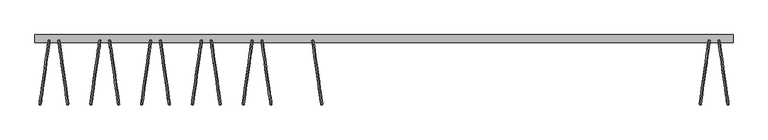
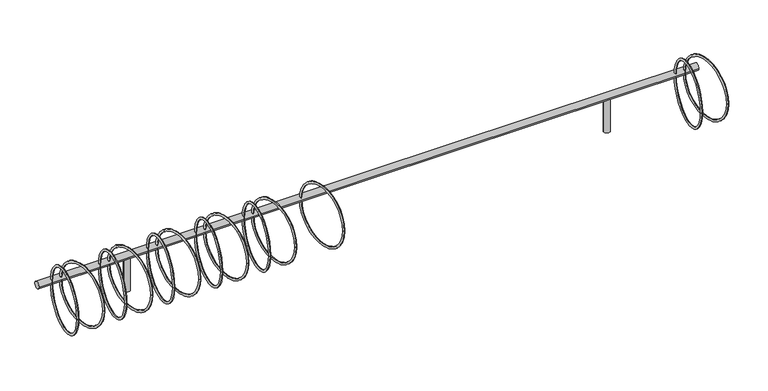
"""IFC4 building model written with IfcOpenShell, lengths in millimetres: geographic element geometry, NLRS_90_SI_WPB_fietsenrek staal_gen_bf : fietsenrek 5500mm 14 plaatsen."""

from ifc_helpers import new_model, si_unit, point, frame, frame_2d, origin, origin_with_axes, place, context, project, spatial, circle_curve, ellipse_curve, trimmed, segment, composite_curve, outline, extrude, source, transform, mapped, element, save
from ifc_brep_helpers import revolved_surface, advanced_brep


def geographic_element_d13230c3(model_context):
    return source(origin(), model_context, "Body", "SolidModel", [
        advanced_brep(
        [(-560.5888305, -21.9255981, 304.7993564), (-492.0982681, -509.2612714, 304.7993564), (-489.8888952, -524.981777, 304.7993564), (-562.7982034, -6.2050925, 304.7993564)],
        [
            (0, 1, circle_curve(frame((-526.3435493, -265.5934347, 304.7993564), z_axis=(0.9902680687415715, 0.1391731009600577, 0.0), x_axis=(0.1391731009600577, -0.9902680687415715, 0.0)), 246.0625)),
            (1, 2, circle_curve(frame((-490.9935817, -517.1215242, 304.7993564), z_axis=(0.0, 0.0, 1.0), x_axis=(-0.13917310096005775, 0.9902680687415715, 0.0)), 7.9375)),
            (2, 3, circle_curve(frame((-526.3435493, -265.5934347, 304.7993564), z_axis=(-0.9902680687415715, -0.1391731009600577, 0.0), x_axis=(0.1391731009600577, -0.9902680687415715, 0.0)), 261.9375)),
            (3, 0, circle_curve(frame((-561.6935169, -14.0653453, 304.7993564), z_axis=(0.0, 0.0, 1.0), x_axis=(0.13917310096005764, -0.9902680687415715, 0.0)), 7.9375)),
            (2, 1, circle_curve(frame((-490.9935817, -517.1215242, 304.7993564), z_axis=(0.0, 0.0, 1.0), x_axis=(-0.13917310096005775, 0.9902680687415715, 0.0)), 7.9375)),
            (0, 3, circle_curve(frame((-561.6935169, -14.0653453, 304.7993564), z_axis=(0.0, 0.0, 1.0), x_axis=(0.13917310096005764, -0.9902680687415715, 0.0)), 7.9375)),
            (1, 0, circle_curve(frame((-526.3435493, -265.5934347, 304.7993564), z_axis=(0.9902680687415715, 0.1391731009600577, 0.0), x_axis=(-0.1391731009600577, 0.9902680687415715, 0.0)), 246.0625)),
            (3, 2, circle_curve(frame((-526.3435493, -265.5934347, 304.7993564), z_axis=(-0.9902680687415715, -0.1391731009600577, 0.0), x_axis=(-0.1391731009600577, 0.9902680687415715, 0.0)), 261.9375)),
        ],
        [
            revolved_surface(trimmed(ellipse_curve(frame((-490.9935817, -517.1215242, 304.7993564), z_axis=(0.0, 0.0, -1.0), x_axis=(-0.13917310096005775, 0.9902680687415715, 0.0)), 7.9375, 7.9375), [point((-489.8888952, -524.981777, 304.7993564))], [point((-492.0982681, -509.2612714, 304.7993564))], True, "CARTESIAN"), (-714.9896164, -292.1059105, 304.7993564), (-0.9902680687415715, -0.1391731009600577, 0.0)),
            revolved_surface(trimmed(ellipse_curve(frame((-490.9935817, -517.1215242, 304.7993564), z_axis=(0.0, 0.0, -1.0), x_axis=(-0.13917310096005775, 0.9902680687415715, 0.0)), 7.9375, 7.9375), [point((-492.0982681, -509.2612714, 304.7993564))], [point((-489.8888952, -524.981777, 304.7993564))], True, "CARTESIAN"), (-714.9896164, -292.1059105, 304.7993564), (-0.9902680687415715, -0.1391731009600577, 0.0)),
            revolved_surface(trimmed(ellipse_curve(frame((-561.6935169, -14.0653453, 304.7993564), z_axis=(0.0, 0.0, 1.0), x_axis=(0.1391731009600577, -0.9902680687415715, 0.0)), 7.9375, 7.9375), [point((-562.7982034, -6.2050925, 304.7993564))], [point((-560.5888305, -21.9255981, 304.7993564))], True, "CARTESIAN"), (-714.9896164, -292.1059105, 304.7993564), (-0.9902680687415715, -0.1391731009600577, 0.0)),
            revolved_surface(trimmed(ellipse_curve(frame((-561.6935169, -14.0653453, 304.7993564), z_axis=(0.0, 0.0, 1.0), x_axis=(0.1391731009600577, -0.9902680687415715, 0.0)), 7.9375, 7.9375), [point((-560.5888305, -21.9255981, 304.7993564))], [point((-562.7982034, -6.2050925, 304.7993564))], True, "CARTESIAN"), (-714.9896164, -292.1059105, 304.7993564), (-0.9902680687415715, -0.1391731009600577, 0.0)),
        ],
        [
            (0, [[1, 2, 3, 4]]),
            (1, [[-3, 5, -1, 6]]),
            (2, [[7, -4, 8, -2]]),
            (3, [[-8, -6, -7, -5]]),
        ],
    ),
        advanced_brep(
        [(-1039.4111695, -21.9255981, 304.7993564), (-1107.9017319, -509.2612714, 304.7993564), (-1110.1111048, -524.981777, 304.7993564), (-1037.2017966, -6.2050925, 304.7993564)],
        [
            (0, 1, circle_curve(frame((-1073.6564507, -265.5934347, 304.7993564), z_axis=(0.990268068741571, -0.13917310096006058, 0.0), x_axis=(-0.13917310096006058, -0.990268068741571, 0.0)), 246.0625)),
            (1, 2, circle_curve(frame((-1109.0064183, -517.1215242, 304.7993564), z_axis=(0.0, 0.0, 1.0), x_axis=(0.13917310096006055, 0.990268068741571, 0.0)), 7.9375)),
            (2, 3, circle_curve(frame((-1073.6564507, -265.5934347, 304.7993564), z_axis=(-0.990268068741571, 0.13917310096006058, 0.0), x_axis=(-0.13917310096006058, -0.990268068741571, 0.0)), 261.9375)),
            (3, 0, circle_curve(frame((-1038.3064831, -14.0653453, 304.7993564), z_axis=(0.0, 0.0, 1.0), x_axis=(-0.1391731009600606, -0.990268068741571, 0.0)), 7.9375)),
            (2, 1, circle_curve(frame((-1109.0064183, -517.1215242, 304.7993564), z_axis=(0.0, 0.0, 1.0), x_axis=(0.13917310096006055, 0.990268068741571, 0.0)), 7.9375)),
            (0, 3, circle_curve(frame((-1038.3064831, -14.0653453, 304.7993564), z_axis=(0.0, 0.0, 1.0), x_axis=(-0.1391731009600606, -0.990268068741571, 0.0)), 7.9375)),
            (1, 0, circle_curve(frame((-1073.6564507, -265.5934347, 304.7993564), z_axis=(0.990268068741571, -0.13917310096006058, 0.0), x_axis=(0.13917310096006058, 0.990268068741571, 0.0)), 246.0625)),
            (3, 2, circle_curve(frame((-1073.6564507, -265.5934347, 304.7993564), z_axis=(-0.990268068741571, 0.13917310096006058, 0.0), x_axis=(0.13917310096006058, 0.990268068741571, 0.0)), 261.9375)),
        ],
        [
            revolved_surface(trimmed(ellipse_curve(frame((-1109.0064183, -517.1215242, 304.7993564), z_axis=(0.0, 0.0, -1.0), x_axis=(0.13917310096006055, 0.990268068741571, 0.0)), 7.9375, 7.9375), [point((-1110.1111048, -524.981777, 304.7993564))], [point((-1107.9017319, -509.2612714, 304.7993564))], True, "CARTESIAN"), (-885.0103836, -292.1059105, 304.7993564), (-0.990268068741571, 0.13917310096006058, 0.0)),
            revolved_surface(trimmed(ellipse_curve(frame((-1109.0064183, -517.1215242, 304.7993564), z_axis=(0.0, 0.0, -1.0), x_axis=(0.13917310096006055, 0.990268068741571, 0.0)), 7.9375, 7.9375), [point((-1107.9017319, -509.2612714, 304.7993564))], [point((-1110.1111048, -524.981777, 304.7993564))], True, "CARTESIAN"), (-885.0103836, -292.1059105, 304.7993564), (-0.990268068741571, 0.13917310096006058, 0.0)),
            revolved_surface(trimmed(ellipse_curve(frame((-1038.3064831, -14.0653453, 304.7993564), z_axis=(0.0, 0.0, 1.0), x_axis=(-0.13917310096006055, -0.990268068741571, 0.0)), 7.9375, 7.9375), [point((-1037.2017966, -6.2050925, 304.7993564))], [point((-1039.4111695, -21.9255981, 304.7993564))], True, "CARTESIAN"), (-885.0103836, -292.1059105, 304.7993564), (-0.990268068741571, 0.13917310096006058, 0.0)),
            revolved_surface(trimmed(ellipse_curve(frame((-1038.3064831, -14.0653453, 304.7993564), z_axis=(0.0, 0.0, 1.0), x_axis=(-0.13917310096006055, -0.990268068741571, 0.0)), 7.9375, 7.9375), [point((-1039.4111695, -21.9255981, 304.7993564))], [point((-1037.2017966, -6.2050925, 304.7993564))], True, "CARTESIAN"), (-885.0103836, -292.1059105, 304.7993564), (-0.990268068741571, 0.13917310096006058, 0.0)),
        ],
        [
            (0, [[1, 2, 3, 4]]),
            (1, [[-3, 5, -1, 6]]),
            (2, [[7, -4, 8, -2]]),
            (3, [[-8, -6, -7, -5]]),
        ],
    ),
        advanced_brep(
        [(-960.5888305, -21.9255981, 304.7993564), (-892.0982681, -509.2612714, 304.7993564), (-889.8888952, -524.981777, 304.7993564), (-962.7982034, -6.2050925, 304.7993564)],
        [
            (0, 1, circle_curve(frame((-926.3435493, -265.5934347, 304.7993564), z_axis=(0.9902680687415715, 0.1391731009600577, 0.0), x_axis=(0.1391731009600577, -0.9902680687415715, 0.0)), 246.0625)),
            (1, 2, circle_curve(frame((-890.9935817, -517.1215242, 304.7993564), z_axis=(0.0, 0.0, 1.0), x_axis=(-0.13917310096005775, 0.9902680687415715, 0.0)), 7.9375)),
            (2, 3, circle_curve(frame((-926.3435493, -265.5934347, 304.7993564), z_axis=(-0.9902680687415715, -0.1391731009600577, 0.0), x_axis=(0.1391731009600577, -0.9902680687415715, 0.0)), 261.9375)),
            (3, 0, circle_curve(frame((-961.6935169, -14.0653453, 304.7993564), z_axis=(0.0, 0.0, 1.0), x_axis=(0.13917310096005764, -0.9902680687415715, 0.0)), 7.9375)),
            (2, 1, circle_curve(frame((-890.9935817, -517.1215242, 304.7993564), z_axis=(0.0, 0.0, 1.0), x_axis=(-0.13917310096005775, 0.9902680687415715, 0.0)), 7.9375)),
            (0, 3, circle_curve(frame((-961.6935169, -14.0653453, 304.7993564), z_axis=(0.0, 0.0, 1.0), x_axis=(0.13917310096005764, -0.9902680687415715, 0.0)), 7.9375)),
            (1, 0, circle_curve(frame((-926.3435493, -265.5934347, 304.7993564), z_axis=(0.9902680687415715, 0.1391731009600577, 0.0), x_axis=(-0.1391731009600577, 0.9902680687415715, 0.0)), 246.0625)),
            (3, 2, circle_curve(frame((-926.3435493, -265.5934347, 304.7993564), z_axis=(-0.9902680687415715, -0.1391731009600577, 0.0), x_axis=(-0.1391731009600577, 0.9902680687415715, 0.0)), 261.9375)),
        ],
        [
            revolved_surface(trimmed(ellipse_curve(frame((-890.9935817, -517.1215242, 304.7993564), z_axis=(0.0, 0.0, -1.0), x_axis=(-0.13917310096005775, 0.9902680687415715, 0.0)), 7.9375, 7.9375), [point((-889.8888952, -524.981777, 304.7993564))], [point((-892.0982681, -509.2612714, 304.7993564))], True, "CARTESIAN"), (-1114.9896164, -292.1059105, 304.7993564), (-0.9902680687415715, -0.1391731009600577, 0.0)),
            revolved_surface(trimmed(ellipse_curve(frame((-890.9935817, -517.1215242, 304.7993564), z_axis=(0.0, 0.0, -1.0), x_axis=(-0.13917310096005775, 0.9902680687415715, 0.0)), 7.9375, 7.9375), [point((-892.0982681, -509.2612714, 304.7993564))], [point((-889.8888952, -524.981777, 304.7993564))], True, "CARTESIAN"), (-1114.9896164, -292.1059105, 304.7993564), (-0.9902680687415715, -0.1391731009600577, 0.0)),
            revolved_surface(trimmed(ellipse_curve(frame((-961.6935169, -14.0653453, 304.7993564), z_axis=(0.0, 0.0, 1.0), x_axis=(0.1391731009600577, -0.9902680687415715, 0.0)), 7.9375, 7.9375), [point((-962.7982034, -6.2050925, 304.7993564))], [point((-960.5888305, -21.9255981, 304.7993564))], True, "CARTESIAN"), (-1114.9896164, -292.1059105, 304.7993564), (-0.9902680687415715, -0.1391731009600577, 0.0)),
            revolved_surface(trimmed(ellipse_curve(frame((-961.6935169, -14.0653453, 304.7993564), z_axis=(0.0, 0.0, 1.0), x_axis=(0.1391731009600577, -0.9902680687415715, 0.0)), 7.9375, 7.9375), [point((-960.5888305, -21.9255981, 304.7993564))], [point((-962.7982034, -6.2050925, 304.7993564))], True, "CARTESIAN"), (-1114.9896164, -292.1059105, 304.7993564), (-0.9902680687415715, -0.1391731009600577, 0.0)),
        ],
        [
            (0, [[1, 2, 3, 4]]),
            (1, [[-3, 5, -1, 6]]),
            (2, [[7, -4, 8, -2]]),
            (3, [[-8, -6, -7, -5]]),
        ],
    ),
        advanced_brep(
        [(-1439.4111695, -21.9255981, 304.7993564), (-1507.9017319, -509.2612714, 304.7993564), (-1510.1111048, -524.981777, 304.7993564), (-1437.2017966, -6.2050925, 304.7993564)],
        [
            (0, 1, circle_curve(frame((-1473.6564507, -265.5934347, 304.7993564), z_axis=(0.990268068741571, -0.13917310096006058, 0.0), x_axis=(-0.13917310096006058, -0.990268068741571, 0.0)), 246.0625)),
            (1, 2, circle_curve(frame((-1509.0064183, -517.1215242, 304.7993564), z_axis=(0.0, 0.0, 1.0), x_axis=(0.13917310096006055, 0.990268068741571, 0.0)), 7.9375)),
            (2, 3, circle_curve(frame((-1473.6564507, -265.5934347, 304.7993564), z_axis=(-0.990268068741571, 0.13917310096006058, 0.0), x_axis=(-0.13917310096006058, -0.990268068741571, 0.0)), 261.9375)),
            (3, 0, circle_curve(frame((-1438.3064831, -14.0653453, 304.7993564), z_axis=(0.0, 0.0, 1.0), x_axis=(-0.1391731009600606, -0.990268068741571, 0.0)), 7.9375)),
            (2, 1, circle_curve(frame((-1509.0064183, -517.1215242, 304.7993564), z_axis=(0.0, 0.0, 1.0), x_axis=(0.13917310096006055, 0.990268068741571, 0.0)), 7.9375)),
            (0, 3, circle_curve(frame((-1438.3064831, -14.0653453, 304.7993564), z_axis=(0.0, 0.0, 1.0), x_axis=(-0.1391731009600606, -0.990268068741571, 0.0)), 7.9375)),
            (1, 0, circle_curve(frame((-1473.6564507, -265.5934347, 304.7993564), z_axis=(0.990268068741571, -0.13917310096006058, 0.0), x_axis=(0.13917310096006058, 0.990268068741571, 0.0)), 246.0625)),
            (3, 2, circle_curve(frame((-1473.6564507, -265.5934347, 304.7993564), z_axis=(-0.990268068741571, 0.13917310096006058, 0.0), x_axis=(0.13917310096006058, 0.990268068741571, 0.0)), 261.9375)),
        ],
        [
            revolved_surface(trimmed(ellipse_curve(frame((-1509.0064183, -517.1215242, 304.7993564), z_axis=(0.0, 0.0, -1.0), x_axis=(0.13917310096006055, 0.990268068741571, 0.0)), 7.9375, 7.9375), [point((-1510.1111048, -524.981777, 304.7993564))], [point((-1507.9017319, -509.2612714, 304.7993564))], True, "CARTESIAN"), (-1285.0103836, -292.1059105, 304.7993564), (-0.990268068741571, 0.13917310096006058, 0.0)),
            revolved_surface(trimmed(ellipse_curve(frame((-1509.0064183, -517.1215242, 304.7993564), z_axis=(0.0, 0.0, -1.0), x_axis=(0.13917310096006055, 0.990268068741571, 0.0)), 7.9375, 7.9375), [point((-1507.9017319, -509.2612714, 304.7993564))], [point((-1510.1111048, -524.981777, 304.7993564))], True, "CARTESIAN"), (-1285.0103836, -292.1059105, 304.7993564), (-0.990268068741571, 0.13917310096006058, 0.0)),
            revolved_surface(trimmed(ellipse_curve(frame((-1438.3064831, -14.0653453, 304.7993564), z_axis=(0.0, 0.0, 1.0), x_axis=(-0.13917310096006055, -0.990268068741571, 0.0)), 7.9375, 7.9375), [point((-1437.2017966, -6.2050925, 304.7993564))], [point((-1439.4111695, -21.9255981, 304.7993564))], True, "CARTESIAN"), (-1285.0103836, -292.1059105, 304.7993564), (-0.990268068741571, 0.13917310096006058, 0.0)),
            revolved_surface(trimmed(ellipse_curve(frame((-1438.3064831, -14.0653453, 304.7993564), z_axis=(0.0, 0.0, 1.0), x_axis=(-0.13917310096006055, -0.990268068741571, 0.0)), 7.9375, 7.9375), [point((-1439.4111695, -21.9255981, 304.7993564))], [point((-1437.2017966, -6.2050925, 304.7993564))], True, "CARTESIAN"), (-1285.0103836, -292.1059105, 304.7993564), (-0.990268068741571, 0.13917310096006058, 0.0)),
        ],
        [
            (0, [[1, 2, 3, 4]]),
            (1, [[-3, 5, -1, 6]]),
            (2, [[7, -4, 8, -2]]),
            (3, [[-8, -6, -7, -5]]),
        ],
    ),
        advanced_brep(
        [(-1360.5888305, -21.9255981, 304.7993564), (-1292.0982681, -509.2612714, 304.7993564), (-1289.8888952, -524.981777, 304.7993564), (-1362.7982034, -6.2050925, 304.7993564)],
        [
            (0, 1, circle_curve(frame((-1326.3435493, -265.5934347, 304.7993564), z_axis=(0.9902680687415715, 0.1391731009600577, 0.0), x_axis=(0.1391731009600577, -0.9902680687415715, 0.0)), 246.0625)),
            (1, 2, circle_curve(frame((-1290.9935817, -517.1215242, 304.7993564), z_axis=(0.0, 0.0, 1.0), x_axis=(-0.13917310096005775, 0.9902680687415715, 0.0)), 7.9375)),
            (2, 3, circle_curve(frame((-1326.3435493, -265.5934347, 304.7993564), z_axis=(-0.9902680687415715, -0.1391731009600577, 0.0), x_axis=(0.1391731009600577, -0.9902680687415715, 0.0)), 261.9375)),
            (3, 0, circle_curve(frame((-1361.6935169, -14.0653453, 304.7993564), z_axis=(0.0, 0.0, 1.0), x_axis=(0.13917310096005764, -0.9902680687415715, 0.0)), 7.9375)),
            (2, 1, circle_curve(frame((-1290.9935817, -517.1215242, 304.7993564), z_axis=(0.0, 0.0, 1.0), x_axis=(-0.13917310096005775, 0.9902680687415715, 0.0)), 7.9375)),
            (0, 3, circle_curve(frame((-1361.6935169, -14.0653453, 304.7993564), z_axis=(0.0, 0.0, 1.0), x_axis=(0.13917310096005764, -0.9902680687415715, 0.0)), 7.9375)),
            (1, 0, circle_curve(frame((-1326.3435493, -265.5934347, 304.7993564), z_axis=(0.9902680687415715, 0.1391731009600577, 0.0), x_axis=(-0.1391731009600577, 0.9902680687415715, 0.0)), 246.0625)),
            (3, 2, circle_curve(frame((-1326.3435493, -265.5934347, 304.7993564), z_axis=(-0.9902680687415715, -0.1391731009600577, 0.0), x_axis=(-0.1391731009600577, 0.9902680687415715, 0.0)), 261.9375)),
        ],
        [
            revolved_surface(trimmed(ellipse_curve(frame((-1290.9935817, -517.1215242, 304.7993564), z_axis=(0.0, 0.0, -1.0), x_axis=(-0.13917310096005775, 0.9902680687415715, 0.0)), 7.9375, 7.9375), [point((-1289.8888952, -524.981777, 304.7993564))], [point((-1292.0982681, -509.2612714, 304.7993564))], True, "CARTESIAN"), (-1514.9896164, -292.1059105, 304.7993564), (-0.9902680687415715, -0.1391731009600577, 0.0)),
            revolved_surface(trimmed(ellipse_curve(frame((-1290.9935817, -517.1215242, 304.7993564), z_axis=(0.0, 0.0, -1.0), x_axis=(-0.13917310096005775, 0.9902680687415715, 0.0)), 7.9375, 7.9375), [point((-1292.0982681, -509.2612714, 304.7993564))], [point((-1289.8888952, -524.981777, 304.7993564))], True, "CARTESIAN"), (-1514.9896164, -292.1059105, 304.7993564), (-0.9902680687415715, -0.1391731009600577, 0.0)),
            revolved_surface(trimmed(ellipse_curve(frame((-1361.6935169, -14.0653453, 304.7993564), z_axis=(0.0, 0.0, 1.0), x_axis=(0.1391731009600577, -0.9902680687415715, 0.0)), 7.9375, 7.9375), [point((-1362.7982034, -6.2050925, 304.7993564))], [point((-1360.5888305, -21.9255981, 304.7993564))], True, "CARTESIAN"), (-1514.9896164, -292.1059105, 304.7993564), (-0.9902680687415715, -0.1391731009600577, 0.0)),
            revolved_surface(trimmed(ellipse_curve(frame((-1361.6935169, -14.0653453, 304.7993564), z_axis=(0.0, 0.0, 1.0), x_axis=(0.1391731009600577, -0.9902680687415715, 0.0)), 7.9375, 7.9375), [point((-1360.5888305, -21.9255981, 304.7993564))], [point((-1362.7982034, -6.2050925, 304.7993564))], True, "CARTESIAN"), (-1514.9896164, -292.1059105, 304.7993564), (-0.9902680687415715, -0.1391731009600577, 0.0)),
        ],
        [
            (0, [[1, 2, 3, 4]]),
            (1, [[-3, 5, -1, 6]]),
            (2, [[7, -4, 8, -2]]),
            (3, [[-8, -6, -7, -5]]),
        ],
    ),
        advanced_brep(
        [(-1839.4111695, -21.9255981, 304.7993564), (-1907.9017319, -509.2612714, 304.7993564), (-1910.1111048, -524.981777, 304.7993564), (-1837.2017966, -6.2050925, 304.7993564)],
        [
            (0, 1, circle_curve(frame((-1873.6564507, -265.5934347, 304.7993564), z_axis=(0.990268068741571, -0.13917310096006058, 0.0), x_axis=(-0.13917310096006058, -0.990268068741571, 0.0)), 246.0625)),
            (1, 2, circle_curve(frame((-1909.0064183, -517.1215242, 304.7993564), z_axis=(0.0, 0.0, 1.0), x_axis=(0.13917310096006055, 0.990268068741571, 0.0)), 7.9375)),
            (2, 3, circle_curve(frame((-1873.6564507, -265.5934347, 304.7993564), z_axis=(-0.990268068741571, 0.13917310096006058, 0.0), x_axis=(-0.13917310096006058, -0.990268068741571, 0.0)), 261.9375)),
            (3, 0, circle_curve(frame((-1838.3064831, -14.0653453, 304.7993564), z_axis=(0.0, 0.0, 1.0), x_axis=(-0.1391731009600606, -0.990268068741571, 0.0)), 7.9375)),
            (2, 1, circle_curve(frame((-1909.0064183, -517.1215242, 304.7993564), z_axis=(0.0, 0.0, 1.0), x_axis=(0.13917310096006055, 0.990268068741571, 0.0)), 7.9375)),
            (0, 3, circle_curve(frame((-1838.3064831, -14.0653453, 304.7993564), z_axis=(0.0, 0.0, 1.0), x_axis=(-0.1391731009600606, -0.990268068741571, 0.0)), 7.9375)),
            (1, 0, circle_curve(frame((-1873.6564507, -265.5934347, 304.7993564), z_axis=(0.990268068741571, -0.13917310096006058, 0.0), x_axis=(0.13917310096006058, 0.990268068741571, 0.0)), 246.0625)),
            (3, 2, circle_curve(frame((-1873.6564507, -265.5934347, 304.7993564), z_axis=(-0.990268068741571, 0.13917310096006058, 0.0), x_axis=(0.13917310096006058, 0.990268068741571, 0.0)), 261.9375)),
        ],
        [
            revolved_surface(trimmed(ellipse_curve(frame((-1909.0064183, -517.1215242, 304.7993564), z_axis=(0.0, 0.0, -1.0), x_axis=(0.13917310096006055, 0.990268068741571, 0.0)), 7.9375, 7.9375), [point((-1910.1111048, -524.981777, 304.7993564))], [point((-1907.9017319, -509.2612714, 304.7993564))], True, "CARTESIAN"), (-1685.0103836, -292.1059105, 304.7993564), (-0.990268068741571, 0.13917310096006058, 0.0)),
            revolved_surface(trimmed(ellipse_curve(frame((-1909.0064183, -517.1215242, 304.7993564), z_axis=(0.0, 0.0, -1.0), x_axis=(0.13917310096006055, 0.990268068741571, 0.0)), 7.9375, 7.9375), [point((-1907.9017319, -509.2612714, 304.7993564))], [point((-1910.1111048, -524.981777, 304.7993564))], True, "CARTESIAN"), (-1685.0103836, -292.1059105, 304.7993564), (-0.990268068741571, 0.13917310096006058, 0.0)),
            revolved_surface(trimmed(ellipse_curve(frame((-1838.3064831, -14.0653453, 304.7993564), z_axis=(0.0, 0.0, 1.0), x_axis=(-0.13917310096006055, -0.990268068741571, 0.0)), 7.9375, 7.9375), [point((-1837.2017966, -6.2050925, 304.7993564))], [point((-1839.4111695, -21.9255981, 304.7993564))], True, "CARTESIAN"), (-1685.0103836, -292.1059105, 304.7993564), (-0.990268068741571, 0.13917310096006058, 0.0)),
            revolved_surface(trimmed(ellipse_curve(frame((-1838.3064831, -14.0653453, 304.7993564), z_axis=(0.0, 0.0, 1.0), x_axis=(-0.13917310096006055, -0.990268068741571, 0.0)), 7.9375, 7.9375), [point((-1839.4111695, -21.9255981, 304.7993564))], [point((-1837.2017966, -6.2050925, 304.7993564))], True, "CARTESIAN"), (-1685.0103836, -292.1059105, 304.7993564), (-0.990268068741571, 0.13917310096006058, 0.0)),
        ],
        [
            (0, [[1, 2, 3, 4]]),
            (1, [[-3, 5, -1, 6]]),
            (2, [[7, -4, 8, -2]]),
            (3, [[-8, -6, -7, -5]]),
        ],
    ),
        advanced_brep(
        [(-1760.5888305, -21.9255981, 304.7993564), (-1692.0982681, -509.2612714, 304.7993564), (-1689.8888952, -524.981777, 304.7993564), (-1762.7982034, -6.2050925, 304.7993564)],
        [
            (0, 1, circle_curve(frame((-1726.3435493, -265.5934347, 304.7993564), z_axis=(0.9902680687415715, 0.1391731009600577, 0.0), x_axis=(0.1391731009600577, -0.9902680687415715, 0.0)), 246.0625)),
            (1, 2, circle_curve(frame((-1690.9935817, -517.1215242, 304.7993564), z_axis=(0.0, 0.0, 1.0), x_axis=(-0.13917310096005775, 0.9902680687415715, 0.0)), 7.9375)),
            (2, 3, circle_curve(frame((-1726.3435493, -265.5934347, 304.7993564), z_axis=(-0.9902680687415715, -0.1391731009600577, 0.0), x_axis=(0.1391731009600577, -0.9902680687415715, 0.0)), 261.9375)),
            (3, 0, circle_curve(frame((-1761.6935169, -14.0653453, 304.7993564), z_axis=(0.0, 0.0, 1.0), x_axis=(0.13917310096005764, -0.9902680687415715, 0.0)), 7.9375)),
            (2, 1, circle_curve(frame((-1690.9935817, -517.1215242, 304.7993564), z_axis=(0.0, 0.0, 1.0), x_axis=(-0.13917310096005775, 0.9902680687415715, 0.0)), 7.9375)),
            (0, 3, circle_curve(frame((-1761.6935169, -14.0653453, 304.7993564), z_axis=(0.0, 0.0, 1.0), x_axis=(0.13917310096005764, -0.9902680687415715, 0.0)), 7.9375)),
            (1, 0, circle_curve(frame((-1726.3435493, -265.5934347, 304.7993564), z_axis=(0.9902680687415715, 0.1391731009600577, 0.0), x_axis=(-0.1391731009600577, 0.9902680687415715, 0.0)), 246.0625)),
            (3, 2, circle_curve(frame((-1726.3435493, -265.5934347, 304.7993564), z_axis=(-0.9902680687415715, -0.1391731009600577, 0.0), x_axis=(-0.1391731009600577, 0.9902680687415715, 0.0)), 261.9375)),
        ],
        [
            revolved_surface(trimmed(ellipse_curve(frame((-1690.9935817, -517.1215242, 304.7993564), z_axis=(0.0, 0.0, -1.0), x_axis=(-0.13917310096005775, 0.9902680687415715, 0.0)), 7.9375, 7.9375), [point((-1689.8888952, -524.981777, 304.7993564))], [point((-1692.0982681, -509.2612714, 304.7993564))], True, "CARTESIAN"), (-1914.9896164, -292.1059105, 304.7993564), (-0.9902680687415715, -0.1391731009600577, 0.0)),
            revolved_surface(trimmed(ellipse_curve(frame((-1690.9935817, -517.1215242, 304.7993564), z_axis=(0.0, 0.0, -1.0), x_axis=(-0.13917310096005775, 0.9902680687415715, 0.0)), 7.9375, 7.9375), [point((-1692.0982681, -509.2612714, 304.7993564))], [point((-1689.8888952, -524.981777, 304.7993564))], True, "CARTESIAN"), (-1914.9896164, -292.1059105, 304.7993564), (-0.9902680687415715, -0.1391731009600577, 0.0)),
            revolved_surface(trimmed(ellipse_curve(frame((-1761.6935169, -14.0653453, 304.7993564), z_axis=(0.0, 0.0, 1.0), x_axis=(0.1391731009600577, -0.9902680687415715, 0.0)), 7.9375, 7.9375), [point((-1762.7982034, -6.2050925, 304.7993564))], [point((-1760.5888305, -21.9255981, 304.7993564))], True, "CARTESIAN"), (-1914.9896164, -292.1059105, 304.7993564), (-0.9902680687415715, -0.1391731009600577, 0.0)),
            revolved_surface(trimmed(ellipse_curve(frame((-1761.6935169, -14.0653453, 304.7993564), z_axis=(0.0, 0.0, 1.0), x_axis=(0.1391731009600577, -0.9902680687415715, 0.0)), 7.9375, 7.9375), [point((-1760.5888305, -21.9255981, 304.7993564))], [point((-1762.7982034, -6.2050925, 304.7993564))], True, "CARTESIAN"), (-1914.9896164, -292.1059105, 304.7993564), (-0.9902680687415715, -0.1391731009600577, 0.0)),
        ],
        [
            (0, [[1, 2, 3, 4]]),
            (1, [[-3, 5, -1, 6]]),
            (2, [[7, -4, 8, -2]]),
            (3, [[-8, -6, -7, -5]]),
        ],
    ),
        advanced_brep(
        [(-2239.4111695, -21.9255981, 304.7993564), (-2307.9017319, -509.2612714, 304.7993564), (-2310.1111048, -524.981777, 304.7993564), (-2237.2017966, -6.2050925, 304.7993564)],
        [
            (0, 1, circle_curve(frame((-2273.6564507, -265.5934347, 304.7993564), z_axis=(0.990268068741571, -0.13917310096006058, 0.0), x_axis=(-0.13917310096006058, -0.990268068741571, 0.0)), 246.0625)),
            (1, 2, circle_curve(frame((-2309.0064183, -517.1215242, 304.7993564), z_axis=(0.0, 0.0, 1.0), x_axis=(0.13917310096006055, 0.990268068741571, 0.0)), 7.9375)),
            (2, 3, circle_curve(frame((-2273.6564507, -265.5934347, 304.7993564), z_axis=(-0.990268068741571, 0.13917310096006058, 0.0), x_axis=(-0.13917310096006058, -0.990268068741571, 0.0)), 261.9375)),
            (3, 0, circle_curve(frame((-2238.3064831, -14.0653453, 304.7993564), z_axis=(0.0, 0.0, 1.0), x_axis=(-0.1391731009600606, -0.990268068741571, 0.0)), 7.9375)),
            (2, 1, circle_curve(frame((-2309.0064183, -517.1215242, 304.7993564), z_axis=(0.0, 0.0, 1.0), x_axis=(0.13917310096006055, 0.990268068741571, 0.0)), 7.9375)),
            (0, 3, circle_curve(frame((-2238.3064831, -14.0653453, 304.7993564), z_axis=(0.0, 0.0, 1.0), x_axis=(-0.1391731009600606, -0.990268068741571, 0.0)), 7.9375)),
            (1, 0, circle_curve(frame((-2273.6564507, -265.5934347, 304.7993564), z_axis=(0.990268068741571, -0.13917310096006058, 0.0), x_axis=(0.13917310096006058, 0.990268068741571, 0.0)), 246.0625)),
            (3, 2, circle_curve(frame((-2273.6564507, -265.5934347, 304.7993564), z_axis=(-0.990268068741571, 0.13917310096006058, 0.0), x_axis=(0.13917310096006058, 0.990268068741571, 0.0)), 261.9375)),
        ],
        [
            revolved_surface(trimmed(ellipse_curve(frame((-2309.0064183, -517.1215242, 304.7993564), z_axis=(0.0, 0.0, -1.0), x_axis=(0.13917310096006055, 0.990268068741571, 0.0)), 7.9375, 7.9375), [point((-2310.1111048, -524.981777, 304.7993564))], [point((-2307.9017319, -509.2612714, 304.7993564))], True, "CARTESIAN"), (-2085.0103836, -292.1059105, 304.7993564), (-0.990268068741571, 0.13917310096006058, 0.0)),
            revolved_surface(trimmed(ellipse_curve(frame((-2309.0064183, -517.1215242, 304.7993564), z_axis=(0.0, 0.0, -1.0), x_axis=(0.13917310096006055, 0.990268068741571, 0.0)), 7.9375, 7.9375), [point((-2307.9017319, -509.2612714, 304.7993564))], [point((-2310.1111048, -524.981777, 304.7993564))], True, "CARTESIAN"), (-2085.0103836, -292.1059105, 304.7993564), (-0.990268068741571, 0.13917310096006058, 0.0)),
            revolved_surface(trimmed(ellipse_curve(frame((-2238.3064831, -14.0653453, 304.7993564), z_axis=(0.0, 0.0, 1.0), x_axis=(-0.13917310096006055, -0.990268068741571, 0.0)), 7.9375, 7.9375), [point((-2237.2017966, -6.2050925, 304.7993564))], [point((-2239.4111695, -21.9255981, 304.7993564))], True, "CARTESIAN"), (-2085.0103836, -292.1059105, 304.7993564), (-0.990268068741571, 0.13917310096006058, 0.0)),
            revolved_surface(trimmed(ellipse_curve(frame((-2238.3064831, -14.0653453, 304.7993564), z_axis=(0.0, 0.0, 1.0), x_axis=(-0.13917310096006055, -0.990268068741571, 0.0)), 7.9375, 7.9375), [point((-2239.4111695, -21.9255981, 304.7993564))], [point((-2237.2017966, -6.2050925, 304.7993564))], True, "CARTESIAN"), (-2085.0103836, -292.1059105, 304.7993564), (-0.990268068741571, 0.13917310096006058, 0.0)),
        ],
        [
            (0, [[1, 2, 3, 4]]),
            (1, [[-3, 5, -1, 6]]),
            (2, [[7, -4, 8, -2]]),
            (3, [[-8, -6, -7, -5]]),
        ],
    ),
        advanced_brep(
        [(-2160.5888305, -21.9255981, 304.7993564), (-2092.0982681, -509.2612714, 304.7993564), (-2089.8888952, -524.981777, 304.7993564), (-2162.7982034, -6.2050925, 304.7993564)],
        [
            (0, 1, circle_curve(frame((-2126.3435493, -265.5934347, 304.7993564), z_axis=(0.9902680687415715, 0.1391731009600577, 0.0), x_axis=(0.1391731009600577, -0.9902680687415715, 0.0)), 246.0625)),
            (1, 2, circle_curve(frame((-2090.9935817, -517.1215242, 304.7993564), z_axis=(0.0, 0.0, 1.0), x_axis=(-0.13917310096005775, 0.9902680687415715, 0.0)), 7.9375)),
            (2, 3, circle_curve(frame((-2126.3435493, -265.5934347, 304.7993564), z_axis=(-0.9902680687415715, -0.1391731009600577, 0.0), x_axis=(0.1391731009600577, -0.9902680687415715, 0.0)), 261.9375)),
            (3, 0, circle_curve(frame((-2161.6935169, -14.0653453, 304.7993564), z_axis=(0.0, 0.0, 1.0), x_axis=(0.13917310096005764, -0.9902680687415715, 0.0)), 7.9375)),
            (2, 1, circle_curve(frame((-2090.9935817, -517.1215242, 304.7993564), z_axis=(0.0, 0.0, 1.0), x_axis=(-0.13917310096005775, 0.9902680687415715, 0.0)), 7.9375)),
            (0, 3, circle_curve(frame((-2161.6935169, -14.0653453, 304.7993564), z_axis=(0.0, 0.0, 1.0), x_axis=(0.13917310096005764, -0.9902680687415715, 0.0)), 7.9375)),
            (1, 0, circle_curve(frame((-2126.3435493, -265.5934347, 304.7993564), z_axis=(0.9902680687415715, 0.1391731009600577, 0.0), x_axis=(-0.1391731009600577, 0.9902680687415715, 0.0)), 246.0625)),
            (3, 2, circle_curve(frame((-2126.3435493, -265.5934347, 304.7993564), z_axis=(-0.9902680687415715, -0.1391731009600577, 0.0), x_axis=(-0.1391731009600577, 0.9902680687415715, 0.0)), 261.9375)),
        ],
        [
            revolved_surface(trimmed(ellipse_curve(frame((-2090.9935817, -517.1215242, 304.7993564), z_axis=(0.0, 0.0, -1.0), x_axis=(-0.13917310096005775, 0.9902680687415715, 0.0)), 7.9375, 7.9375), [point((-2089.8888952, -524.981777, 304.7993564))], [point((-2092.0982681, -509.2612714, 304.7993564))], True, "CARTESIAN"), (-2314.9896164, -292.1059105, 304.7993564), (-0.9902680687415715, -0.1391731009600577, 0.0)),
            revolved_surface(trimmed(ellipse_curve(frame((-2090.9935817, -517.1215242, 304.7993564), z_axis=(0.0, 0.0, -1.0), x_axis=(-0.13917310096005775, 0.9902680687415715, 0.0)), 7.9375, 7.9375), [point((-2092.0982681, -509.2612714, 304.7993564))], [point((-2089.8888952, -524.981777, 304.7993564))], True, "CARTESIAN"), (-2314.9896164, -292.1059105, 304.7993564), (-0.9902680687415715, -0.1391731009600577, 0.0)),
            revolved_surface(trimmed(ellipse_curve(frame((-2161.6935169, -14.0653453, 304.7993564), z_axis=(0.0, 0.0, 1.0), x_axis=(0.1391731009600577, -0.9902680687415715, 0.0)), 7.9375, 7.9375), [point((-2162.7982034, -6.2050925, 304.7993564))], [point((-2160.5888305, -21.9255981, 304.7993564))], True, "CARTESIAN"), (-2314.9896164, -292.1059105, 304.7993564), (-0.9902680687415715, -0.1391731009600577, 0.0)),
            revolved_surface(trimmed(ellipse_curve(frame((-2161.6935169, -14.0653453, 304.7993564), z_axis=(0.0, 0.0, 1.0), x_axis=(0.1391731009600577, -0.9902680687415715, 0.0)), 7.9375, 7.9375), [point((-2160.5888305, -21.9255981, 304.7993564))], [point((-2162.7982034, -6.2050925, 304.7993564))], True, "CARTESIAN"), (-2314.9896164, -292.1059105, 304.7993564), (-0.9902680687415715, -0.1391731009600577, 0.0)),
        ],
        [
            (0, [[1, 2, 3, 4]]),
            (1, [[-3, 5, -1, 6]]),
            (2, [[7, -4, 8, -2]]),
            (3, [[-8, -6, -7, -5]]),
        ],
    ),
        advanced_brep(
        [(2560.5888305, -21.9255981, 304.7993564), (2492.0982681, -509.2612714, 304.7993564), (2489.8888952, -524.981777, 304.7993564), (2562.7982034, -6.2050925, 304.7993564)],
        [
            (0, 1, circle_curve(frame((2526.3435493, -265.5934347, 304.7993564), z_axis=(0.990268068741571, -0.13917310096006058, 0.0), x_axis=(-0.13917310096006058, -0.990268068741571, 0.0)), 246.0625)),
            (1, 2, circle_curve(frame((2490.9935817, -517.1215242, 304.7993564), z_axis=(0.0, 0.0, 1.0), x_axis=(0.13917310096006055, 0.990268068741571, 0.0)), 7.9375)),
            (2, 3, circle_curve(frame((2526.3435493, -265.5934347, 304.7993564), z_axis=(-0.990268068741571, 0.13917310096006058, 0.0), x_axis=(-0.13917310096006058, -0.990268068741571, 0.0)), 261.9375)),
            (3, 0, circle_curve(frame((2561.6935169, -14.0653453, 304.7993564), z_axis=(0.0, 0.0, 1.0), x_axis=(-0.1391731009600606, -0.990268068741571, 0.0)), 7.9375)),
            (2, 1, circle_curve(frame((2490.9935817, -517.1215242, 304.7993564), z_axis=(0.0, 0.0, 1.0), x_axis=(0.13917310096006055, 0.990268068741571, 0.0)), 7.9375)),
            (0, 3, circle_curve(frame((2561.6935169, -14.0653453, 304.7993564), z_axis=(0.0, 0.0, 1.0), x_axis=(-0.1391731009600606, -0.990268068741571, 0.0)), 7.9375)),
            (1, 0, circle_curve(frame((2526.3435493, -265.5934347, 304.7993564), z_axis=(0.990268068741571, -0.13917310096006058, 0.0), x_axis=(0.13917310096006058, 0.990268068741571, 0.0)), 246.0625)),
            (3, 2, circle_curve(frame((2526.3435493, -265.5934347, 304.7993564), z_axis=(-0.990268068741571, 0.13917310096006058, 0.0), x_axis=(0.13917310096006058, 0.990268068741571, 0.0)), 261.9375)),
        ],
        [
            revolved_surface(trimmed(ellipse_curve(frame((2490.9935817, -517.1215242, 304.7993564), z_axis=(0.0, 0.0, -1.0), x_axis=(0.13917310096006055, 0.990268068741571, 0.0)), 7.9375, 7.9375), [point((2489.8888952, -524.981777, 304.7993564))], [point((2492.0982681, -509.2612714, 304.7993564))], True, "CARTESIAN"), (2714.9896164, -292.1059105, 304.7993564), (-0.990268068741571, 0.13917310096006058, 0.0)),
            revolved_surface(trimmed(ellipse_curve(frame((2490.9935817, -517.1215242, 304.7993564), z_axis=(0.0, 0.0, -1.0), x_axis=(0.13917310096006055, 0.990268068741571, 0.0)), 7.9375, 7.9375), [point((2492.0982681, -509.2612714, 304.7993564))], [point((2489.8888952, -524.981777, 304.7993564))], True, "CARTESIAN"), (2714.9896164, -292.1059105, 304.7993564), (-0.990268068741571, 0.13917310096006058, 0.0)),
            revolved_surface(trimmed(ellipse_curve(frame((2561.6935169, -14.0653453, 304.7993564), z_axis=(0.0, 0.0, 1.0), x_axis=(-0.13917310096006055, -0.990268068741571, 0.0)), 7.9375, 7.9375), [point((2562.7982034, -6.2050925, 304.7993564))], [point((2560.5888305, -21.9255981, 304.7993564))], True, "CARTESIAN"), (2714.9896164, -292.1059105, 304.7993564), (-0.990268068741571, 0.13917310096006058, 0.0)),
            revolved_surface(trimmed(ellipse_curve(frame((2561.6935169, -14.0653453, 304.7993564), z_axis=(0.0, 0.0, 1.0), x_axis=(-0.13917310096006055, -0.990268068741571, 0.0)), 7.9375, 7.9375), [point((2560.5888305, -21.9255981, 304.7993564))], [point((2562.7982034, -6.2050925, 304.7993564))], True, "CARTESIAN"), (2714.9896164, -292.1059105, 304.7993564), (-0.990268068741571, 0.13917310096006058, 0.0)),
        ],
        [
            (0, [[1, 2, 3, 4]]),
            (1, [[-3, 5, -1, 6]]),
            (2, [[7, -4, 8, -2]]),
            (3, [[-8, -6, -7, -5]]),
        ],
    ),
        advanced_brep(
        [(2639.4111695, -21.9255981, 304.7993564), (2707.9017319, -509.2612714, 304.7993564), (2710.1111048, -524.981777, 304.7993564), (2637.2017966, -6.2050925, 304.7993564)],
        [
            (0, 1, circle_curve(frame((2673.6564507, -265.5934347, 304.7993564), z_axis=(0.9902680687415715, 0.1391731009600577, 0.0), x_axis=(0.1391731009600577, -0.9902680687415715, 0.0)), 246.0625)),
            (1, 2, circle_curve(frame((2709.0064183, -517.1215242, 304.7993564), z_axis=(0.0, 0.0, 1.0), x_axis=(-0.13917310096005775, 0.9902680687415715, 0.0)), 7.9375)),
            (2, 3, circle_curve(frame((2673.6564507, -265.5934347, 304.7993564), z_axis=(-0.9902680687415715, -0.1391731009600577, 0.0), x_axis=(0.1391731009600577, -0.9902680687415715, 0.0)), 261.9375)),
            (3, 0, circle_curve(frame((2638.3064831, -14.0653453, 304.7993564), z_axis=(0.0, 0.0, 1.0), x_axis=(0.13917310096005764, -0.9902680687415715, 0.0)), 7.9375)),
            (2, 1, circle_curve(frame((2709.0064183, -517.1215242, 304.7993564), z_axis=(0.0, 0.0, 1.0), x_axis=(-0.13917310096005775, 0.9902680687415715, 0.0)), 7.9375)),
            (0, 3, circle_curve(frame((2638.3064831, -14.0653453, 304.7993564), z_axis=(0.0, 0.0, 1.0), x_axis=(0.13917310096005764, -0.9902680687415715, 0.0)), 7.9375)),
            (1, 0, circle_curve(frame((2673.6564507, -265.5934347, 304.7993564), z_axis=(0.9902680687415715, 0.1391731009600577, 0.0), x_axis=(-0.1391731009600577, 0.9902680687415715, 0.0)), 246.0625)),
            (3, 2, circle_curve(frame((2673.6564507, -265.5934347, 304.7993564), z_axis=(-0.9902680687415715, -0.1391731009600577, 0.0), x_axis=(-0.1391731009600577, 0.9902680687415715, 0.0)), 261.9375)),
        ],
        [
            revolved_surface(trimmed(ellipse_curve(frame((2709.0064183, -517.1215242, 304.7993564), z_axis=(0.0, 0.0, -1.0), x_axis=(-0.13917310096005775, 0.9902680687415715, 0.0)), 7.9375, 7.9375), [point((2710.1111048, -524.981777, 304.7993564))], [point((2707.9017319, -509.2612714, 304.7993564))], True, "CARTESIAN"), (2485.0103836, -292.1059105, 304.7993564), (-0.9902680687415715, -0.1391731009600577, 0.0)),
            revolved_surface(trimmed(ellipse_curve(frame((2709.0064183, -517.1215242, 304.7993564), z_axis=(0.0, 0.0, -1.0), x_axis=(-0.13917310096005775, 0.9902680687415715, 0.0)), 7.9375, 7.9375), [point((2707.9017319, -509.2612714, 304.7993564))], [point((2710.1111048, -524.981777, 304.7993564))], True, "CARTESIAN"), (2485.0103836, -292.1059105, 304.7993564), (-0.9902680687415715, -0.1391731009600577, 0.0)),
            revolved_surface(trimmed(ellipse_curve(frame((2638.3064831, -14.0653453, 304.7993564), z_axis=(0.0, 0.0, 1.0), x_axis=(0.1391731009600577, -0.9902680687415715, 0.0)), 7.9375, 7.9375), [point((2637.2017966, -6.2050925, 304.7993564))], [point((2639.4111695, -21.9255981, 304.7993564))], True, "CARTESIAN"), (2485.0103836, -292.1059105, 304.7993564), (-0.9902680687415715, -0.1391731009600577, 0.0)),
            revolved_surface(trimmed(ellipse_curve(frame((2638.3064831, -14.0653453, 304.7993564), z_axis=(0.0, 0.0, 1.0), x_axis=(0.1391731009600577, -0.9902680687415715, 0.0)), 7.9375, 7.9375), [point((2639.4111695, -21.9255981, 304.7993564))], [point((2637.2017966, -6.2050925, 304.7993564))], True, "CARTESIAN"), (2485.0103836, -292.1059105, 304.7993564), (-0.9902680687415715, -0.1391731009600577, 0.0)),
        ],
        [
            (0, [[1, 2, 3, 4]]),
            (1, [[-3, 5, -1, 6]]),
            (2, [[7, -4, 8, -2]]),
            (3, [[-8, -6, -7, -5]]),
        ],
    ),
        advanced_brep(
        [(-2639.4111695, -21.9255981, 304.7993564), (-2707.9017319, -509.2612714, 304.7993564), (-2710.1111048, -524.981777, 304.7993564), (-2637.2017966, -6.2050925, 304.7993564)],
        [
            (0, 1, circle_curve(frame((-2673.6564507, -265.5934347, 304.7993564), z_axis=(0.990268068741571, -0.13917310096006058, 0.0), x_axis=(-0.13917310096006058, -0.990268068741571, 0.0)), 246.0625)),
            (1, 2, circle_curve(frame((-2709.0064183, -517.1215242, 304.7993564), z_axis=(0.0, 0.0, 1.0), x_axis=(0.13917310096006055, 0.990268068741571, 0.0)), 7.9375)),
            (2, 3, circle_curve(frame((-2673.6564507, -265.5934347, 304.7993564), z_axis=(-0.990268068741571, 0.13917310096006058, 0.0), x_axis=(-0.13917310096006058, -0.990268068741571, 0.0)), 261.9375)),
            (3, 0, circle_curve(frame((-2638.3064831, -14.0653453, 304.7993564), z_axis=(0.0, 0.0, 1.0), x_axis=(-0.1391731009600606, -0.990268068741571, 0.0)), 7.9375)),
            (2, 1, circle_curve(frame((-2709.0064183, -517.1215242, 304.7993564), z_axis=(0.0, 0.0, 1.0), x_axis=(0.13917310096006055, 0.990268068741571, 0.0)), 7.9375)),
            (0, 3, circle_curve(frame((-2638.3064831, -14.0653453, 304.7993564), z_axis=(0.0, 0.0, 1.0), x_axis=(-0.1391731009600606, -0.990268068741571, 0.0)), 7.9375)),
            (1, 0, circle_curve(frame((-2673.6564507, -265.5934347, 304.7993564), z_axis=(0.990268068741571, -0.13917310096006058, 0.0), x_axis=(0.13917310096006058, 0.990268068741571, 0.0)), 246.0625)),
            (3, 2, circle_curve(frame((-2673.6564507, -265.5934347, 304.7993564), z_axis=(-0.990268068741571, 0.13917310096006058, 0.0), x_axis=(0.13917310096006058, 0.990268068741571, 0.0)), 261.9375)),
        ],
        [
            revolved_surface(trimmed(ellipse_curve(frame((-2709.0064183, -517.1215242, 304.7993564), z_axis=(0.0, 0.0, -1.0), x_axis=(0.13917310096006055, 0.990268068741571, 0.0)), 7.9375, 7.9375), [point((-2710.1111048, -524.981777, 304.7993564))], [point((-2707.9017319, -509.2612714, 304.7993564))], True, "CARTESIAN"), (-2485.0103836, -292.1059105, 304.7993564), (-0.990268068741571, 0.13917310096006058, 0.0)),
            revolved_surface(trimmed(ellipse_curve(frame((-2709.0064183, -517.1215242, 304.7993564), z_axis=(0.0, 0.0, -1.0), x_axis=(0.13917310096006055, 0.990268068741571, 0.0)), 7.9375, 7.9375), [point((-2707.9017319, -509.2612714, 304.7993564))], [point((-2710.1111048, -524.981777, 304.7993564))], True, "CARTESIAN"), (-2485.0103836, -292.1059105, 304.7993564), (-0.990268068741571, 0.13917310096006058, 0.0)),
            revolved_surface(trimmed(ellipse_curve(frame((-2638.3064831, -14.0653453, 304.7993564), z_axis=(0.0, 0.0, 1.0), x_axis=(-0.13917310096006055, -0.990268068741571, 0.0)), 7.9375, 7.9375), [point((-2637.2017966, -6.2050925, 304.7993564))], [point((-2639.4111695, -21.9255981, 304.7993564))], True, "CARTESIAN"), (-2485.0103836, -292.1059105, 304.7993564), (-0.990268068741571, 0.13917310096006058, 0.0)),
            revolved_surface(trimmed(ellipse_curve(frame((-2638.3064831, -14.0653453, 304.7993564), z_axis=(0.0, 0.0, 1.0), x_axis=(-0.13917310096006055, -0.990268068741571, 0.0)), 7.9375, 7.9375), [point((-2639.4111695, -21.9255981, 304.7993564))], [point((-2637.2017966, -6.2050925, 304.7993564))], True, "CARTESIAN"), (-2485.0103836, -292.1059105, 304.7993564), (-0.990268068741571, 0.13917310096006058, 0.0)),
        ],
        [
            (0, [[1, 2, 3, 4]]),
            (1, [[-3, 5, -1, 6]]),
            (2, [[7, -4, 8, -2]]),
            (3, [[-8, -6, -7, -5]]),
        ],
    ),
        advanced_brep(
        [(-2560.5888305, -21.9255981, 304.7993564), (-2492.0982681, -509.2612714, 304.7993564), (-2489.8888952, -524.981777, 304.7993564), (-2562.7982034, -6.2050925, 304.7993564)],
        [
            (0, 1, circle_curve(frame((-2526.3435493, -265.5934347, 304.7993564), z_axis=(0.9902680687415715, 0.1391731009600577, 0.0), x_axis=(0.1391731009600577, -0.9902680687415715, 0.0)), 246.0625)),
            (1, 2, circle_curve(frame((-2490.9935817, -517.1215242, 304.7993564), z_axis=(0.0, 0.0, 1.0), x_axis=(-0.13917310096005775, 0.9902680687415715, 0.0)), 7.9375)),
            (2, 3, circle_curve(frame((-2526.3435493, -265.5934347, 304.7993564), z_axis=(-0.9902680687415715, -0.1391731009600577, 0.0), x_axis=(0.1391731009600577, -0.9902680687415715, 0.0)), 261.9375)),
            (3, 0, circle_curve(frame((-2561.6935169, -14.0653453, 304.7993564), z_axis=(0.0, 0.0, 1.0), x_axis=(0.13917310096005764, -0.9902680687415715, 0.0)), 7.9375)),
            (2, 1, circle_curve(frame((-2490.9935817, -517.1215242, 304.7993564), z_axis=(0.0, 0.0, 1.0), x_axis=(-0.13917310096005775, 0.9902680687415715, 0.0)), 7.9375)),
            (0, 3, circle_curve(frame((-2561.6935169, -14.0653453, 304.7993564), z_axis=(0.0, 0.0, 1.0), x_axis=(0.13917310096005764, -0.9902680687415715, 0.0)), 7.9375)),
            (1, 0, circle_curve(frame((-2526.3435493, -265.5934347, 304.7993564), z_axis=(0.9902680687415715, 0.1391731009600577, 0.0), x_axis=(-0.1391731009600577, 0.9902680687415715, 0.0)), 246.0625)),
            (3, 2, circle_curve(frame((-2526.3435493, -265.5934347, 304.7993564), z_axis=(-0.9902680687415715, -0.1391731009600577, 0.0), x_axis=(-0.1391731009600577, 0.9902680687415715, 0.0)), 261.9375)),
        ],
        [
            revolved_surface(trimmed(ellipse_curve(frame((-2490.9935817, -517.1215242, 304.7993564), z_axis=(0.0, 0.0, -1.0), x_axis=(-0.13917310096005775, 0.9902680687415715, 0.0)), 7.9375, 7.9375), [point((-2489.8888952, -524.981777, 304.7993564))], [point((-2492.0982681, -509.2612714, 304.7993564))], True, "CARTESIAN"), (-2714.9896164, -292.1059105, 304.7993564), (-0.9902680687415715, -0.1391731009600577, 0.0)),
            revolved_surface(trimmed(ellipse_curve(frame((-2490.9935817, -517.1215242, 304.7993564), z_axis=(0.0, 0.0, -1.0), x_axis=(-0.13917310096005775, 0.9902680687415715, 0.0)), 7.9375, 7.9375), [point((-2492.0982681, -509.2612714, 304.7993564))], [point((-2489.8888952, -524.981777, 304.7993564))], True, "CARTESIAN"), (-2714.9896164, -292.1059105, 304.7993564), (-0.9902680687415715, -0.1391731009600577, 0.0)),
            revolved_surface(trimmed(ellipse_curve(frame((-2561.6935169, -14.0653453, 304.7993564), z_axis=(0.0, 0.0, 1.0), x_axis=(0.1391731009600577, -0.9902680687415715, 0.0)), 7.9375, 7.9375), [point((-2562.7982034, -6.2050925, 304.7993564))], [point((-2560.5888305, -21.9255981, 304.7993564))], True, "CARTESIAN"), (-2714.9896164, -292.1059105, 304.7993564), (-0.9902680687415715, -0.1391731009600577, 0.0)),
            revolved_surface(trimmed(ellipse_curve(frame((-2561.6935169, -14.0653453, 304.7993564), z_axis=(0.0, 0.0, 1.0), x_axis=(0.1391731009600577, -0.9902680687415715, 0.0)), 7.9375, 7.9375), [point((-2560.5888305, -21.9255981, 304.7993564))], [point((-2562.7982034, -6.2050925, 304.7993564))], True, "CARTESIAN"), (-2714.9896164, -292.1059105, 304.7993564), (-0.9902680687415715, -0.1391731009600577, 0.0)),
        ],
        [
            (0, [[1, 2, 3, 4]]),
            (1, [[-3, 5, -1, 6]]),
            (2, [[7, -4, 8, -2]]),
            (3, [[-8, -6, -7, -5]]),
        ],
    ),
        extrude(outline(composite_curve([segment(trimmed(circle_curve(frame_2d((2000.0, 0.0)), 25.4), [point((1974.6, 0.0))], [point((2025.4, 0.0))], False, "CARTESIAN"), True, "CONTINUOUS"), segment(trimmed(circle_curve(frame_2d((2000.0, 0.0)), 25.4), [point((2025.4, 0.0))], [point((1974.6, 0.0))], False, "CARTESIAN"), True, "CONTINUOUS")], self_intersect=False)), origin_with_axes(), (0.0, 0.0, 1.0), 304.8),
        extrude(outline(composite_curve([segment(trimmed(circle_curve(frame_2d((2000.0, 0.0)), 25.4), [point((1974.6, 0.0))], [point((2025.4, 0.0))], False, "CARTESIAN"), True, "CONTINUOUS"), segment(trimmed(circle_curve(frame_2d((2000.0, 0.0)), 25.4), [point((2025.4, 0.0))], [point((1974.6, 0.0))], False, "CARTESIAN"), True, "CONTINUOUS")], self_intersect=False)), origin_with_axes(), (0.0, 0.0, 1.0), 304.8),
        extrude(outline(composite_curve([segment(trimmed(circle_curve(frame_2d((-2000.0, 0.0)), 25.4), [point((-2025.4, 0.0))], [point((-1974.6, 0.0))], False, "CARTESIAN"), True, "CONTINUOUS"), segment(trimmed(circle_curve(frame_2d((-2000.0, 0.0)), 25.4), [point((-1974.6, 0.0))], [point((-2025.4, 0.0))], False, "CARTESIAN"), True, "CONTINUOUS")], self_intersect=False)), origin_with_axes(), (0.0, 0.0, 1.0), 304.8),
        extrude(outline(composite_curve([segment(trimmed(circle_curve(frame_2d((0.0, 304.8)), 30.1625), [point((30.1625, 304.8))], [point((-30.1625, 304.8))], False, "CARTESIAN"), True, "CONTINUOUS"), segment(trimmed(circle_curve(frame_2d((0.0, 304.8)), 30.1625), [point((-30.1625, 304.8))], [point((30.1625, 304.8))], False, "CARTESIAN"), True, "CONTINUOUS")], self_intersect=False)), frame((-2750.0, 0.0, 0.0), z_axis=(1.0, 0.0, 0.0), x_axis=(0.0, 1.0, 0.0)), (0.0, 0.0, 1.0), 5500.0),
    ])


if __name__ == "__main__":
    model = new_model("IFC4")
    model_context = context("Model", 3, world=origin())
    ifc_project = project(units=[si_unit("LENGTHUNIT", "METRE", prefix="MILLI")], contexts=[model_context])
    site = spatial("IfcSite", under=ifc_project)
    building = spatial("IfcBuilding", under=site)
    placement = place(None, origin())
    geographic_element_shape = geographic_element_d13230c3(model_context)
    element("IfcGeographicElement", 1, ObjectType="NLRS_90_SI_WPB_fietsenrek staal_gen_bf : fietsenrek 5500mm 14 plaatsen", at=placement, inside=building, context=model_context, shape_type="MappedRepresentation", body=[
        mapped(geographic_element_shape, transform((0.0, 0.0, 0.0), x_axis=(1.0, 0.0, 0.0), y_axis=(0.0, 1.0, 0.0), z_axis=(0.0, 0.0, 1.0))),
    ])
    save(model, "model.ifc")

# Revit data of these elements
# Type "NLRS_90_SI_WPB_fietsenrek staal_gen_bf : fietsenrek 5500mm 14 plaatsen"
#   Type IFC Predefined Type = "USERDEFINED"
#   Export Type to IFC As = "IfcGeographicElementType"
#   Type IfcGUID = "1jnPA0m7n0IPwpoVFqyx6D"
#   Assembly Code = "90.81"
#   IfcName[Type] = "fietsenrek 5500mm 14 plaatsen"
#   IfcDescription[Type] = "fietsenrek 6m lengte 2x15 plaatsen"
#   IfcObjectType[Type] = "BICYCLE_RACK"
#   IfcExportAs[Type] = "IfcGeographicElementType"
#   IfcExportType[Type] = "USERDEFINED"
#   Model = "generiek"
#   Manufacturer = "generiek"
#   Description = "fietsenrek 6m lengte 2x15 plaatsen"
#   NLRS_C_lengte = 5500.00 mm
#   NLRS_C_afstand = 4000.00 mm
#   rek_dubbel = no
#   NLRS_C_aantal = 14
#   NLRS_C_materiaal = none
#   Default Elevation = 0
